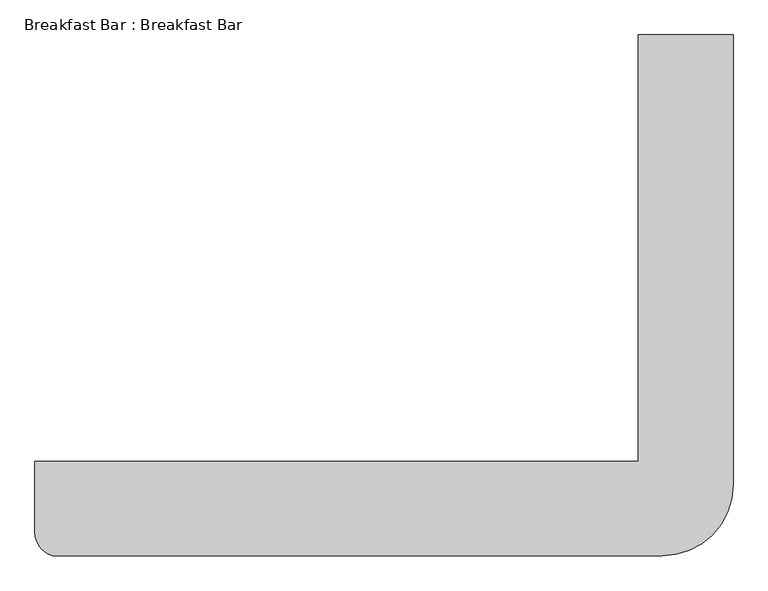
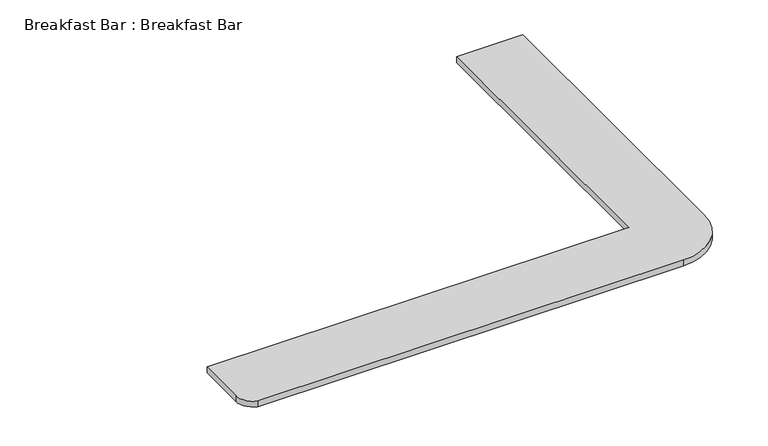
"""IFC4 building model written with IfcOpenShell, lengths in millimetres: furniture geometry, Breakfast Bar : Breakfast Bar."""

from ifc_helpers import new_model, si_unit, point, frame, frame_2d, origin, place, context, project, spatial, polyline, circle_curve, trimmed, segment, composite_curve, outline, extrude, source, transform, mapped, element, save


def breakfast_bar_breakfast_bar_5ef7b973(model_context):
    return source(origin(), model_context, "Body", "SweptSolid", [
        extrude(outline(composite_curve([segment(polyline([(8326.4901433, 8697.9125), (8326.4901433, 10529.8875), (8732.8901433, 10529.8875), (8732.8901433, 8596.3125)]), True, "CONTINUOUS"), segment(trimmed(circle_curve(frame_2d((8428.0901433, 8596.3125)), 304.8), [point((8732.8901433, 8596.3125))], [point((8428.0901433, 8291.5125))], False, "CARTESIAN"), True, "CONTINUOUS"), segment(polyline([(8428.0901433, 8291.5125), (5813.0389296, 8291.5125)]), True, "CONTINUOUS"), segment(trimmed(circle_curve(frame_2d((5841.0918925, 8393.1125)), 105.4017491), [point((5813.0389296, 8291.5125))], [point((5735.6901433, 8393.1125))], False, "CARTESIAN"), True, "CONTINUOUS"), segment(polyline([(5735.6901433, 8393.1125), (5735.6901433, 8697.9125), (8326.4901433, 8697.9125)]), True, "CONTINUOUS")], self_intersect=False)), frame((0.0, 0.0, 1066.8), z_axis=(0.0, 0.0, 1.0), x_axis=(1.0, 0.0, 0.0)), (0.0, 0.0, 1.0), 38.1),
    ])


if __name__ == "__main__":
    model = new_model("IFC4")
    model_context = context("Model", 3, world=origin())
    ifc_project = project(units=[si_unit("LENGTHUNIT", "METRE", prefix="MILLI")], contexts=[model_context])
    site = spatial("IfcSite", under=ifc_project)
    building = spatial("IfcBuilding", under=site)
    placement = place(None, origin())
    breakfast_bar_breakfast_bar_shape = breakfast_bar_breakfast_bar_5ef7b973(model_context)
    element("IfcFurniture", 1, ObjectType="Breakfast Bar : Breakfast Bar", at=placement, inside=building, context=model_context, shape_type="MappedRepresentation", body=[
        mapped(breakfast_bar_breakfast_bar_shape, transform((0.0, 0.0, 0.0), x_axis=(1.0, 0.0, 0.0), y_axis=(0.0, 1.0, 0.0), z_axis=(0.0, 0.0, 1.0))),
    ])
    save(model, "model.ifc")

# Revit data of these elements
# Type "Breakfast Bar : Breakfast Bar"
#   COBie.Type = no
# Element 1 (IfcFurniture, "Breakfast Bar : Breakfast Bar")
#   Materials on its faces: "Corian - Dusk"
# Materials
#   "Corian - Dusk": class "Plastic", colour RGB 75 95 146, transparency 0, Manufacturer = "Corning", Cost = 0
